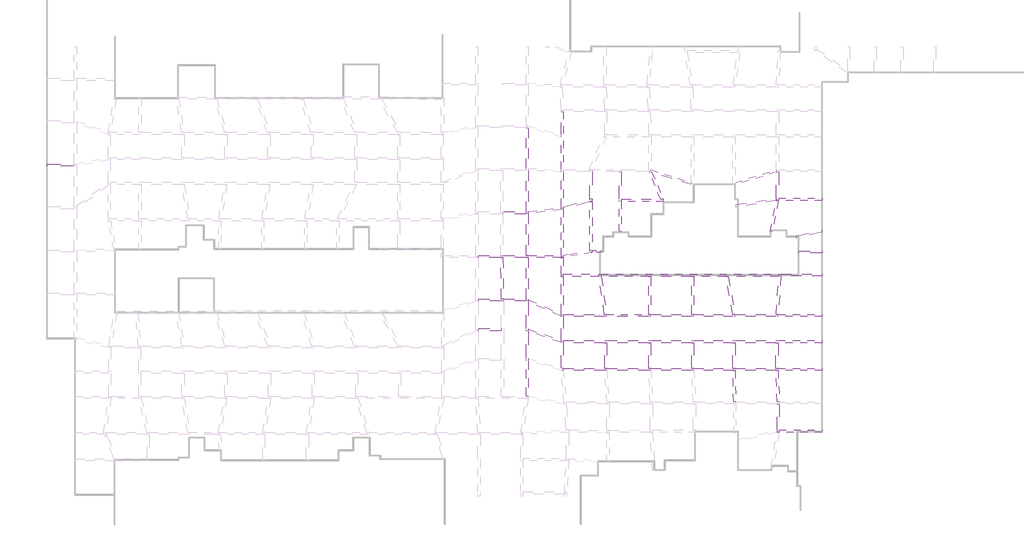
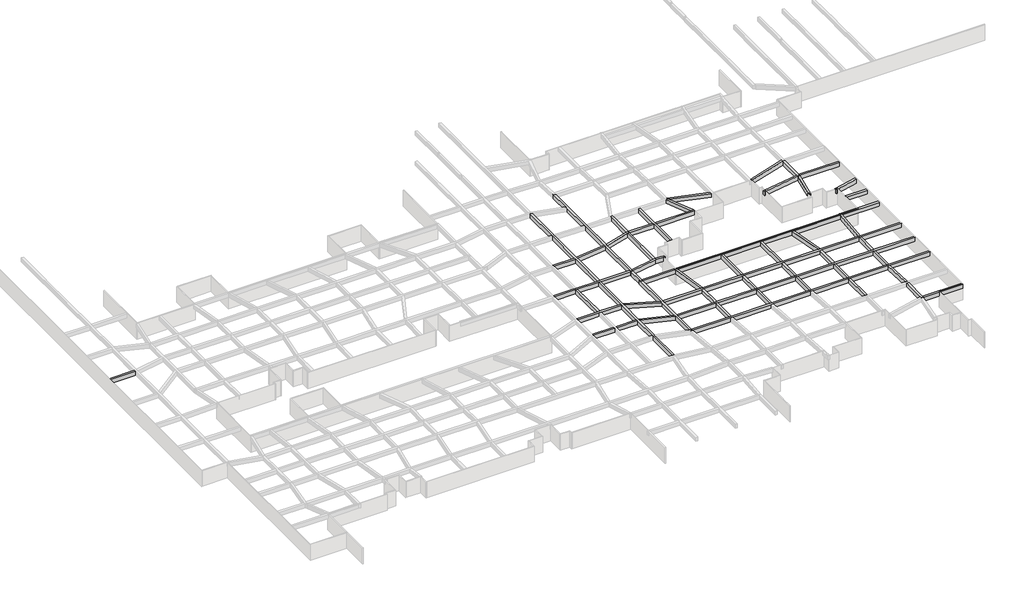
# One storey, part 13 of 45: 50 beams.
# Revit data of these elements (continued)
# Type "混凝土 - 矩形梁 : KL_beam"
#   Length [instance default] = 1524 mm
#   b = 400 mm
#   h = 800 mm
#   Structural Material [instance default] = 混凝土 - 现场浇注混凝土
#   Assembly Code = ""
# Elements 1, 2, 3, 4, 5, 6, 7, 8, 9, 10, 11, 12, 13, 14, 15, 16, 17, 18, 19, 20, 21, 22, 23, 24, 25, 26, 27, 28, 29, 30, 31, 32, 33, 34, 35, 36, 37, 38, 39, 40, 41, 42, 43, 44, 45, 46, 47, 48, 49, 50 (IfcBeam, "混凝土 - 矩形梁 : KL_beam")
#   Comments = ""
#   Structural Material = none
#   Phase Created = 新构造
# Materials
#   "混凝土 - 现场浇注混凝土": class "混凝土", colour RGB 192 192 192, transparency 0
